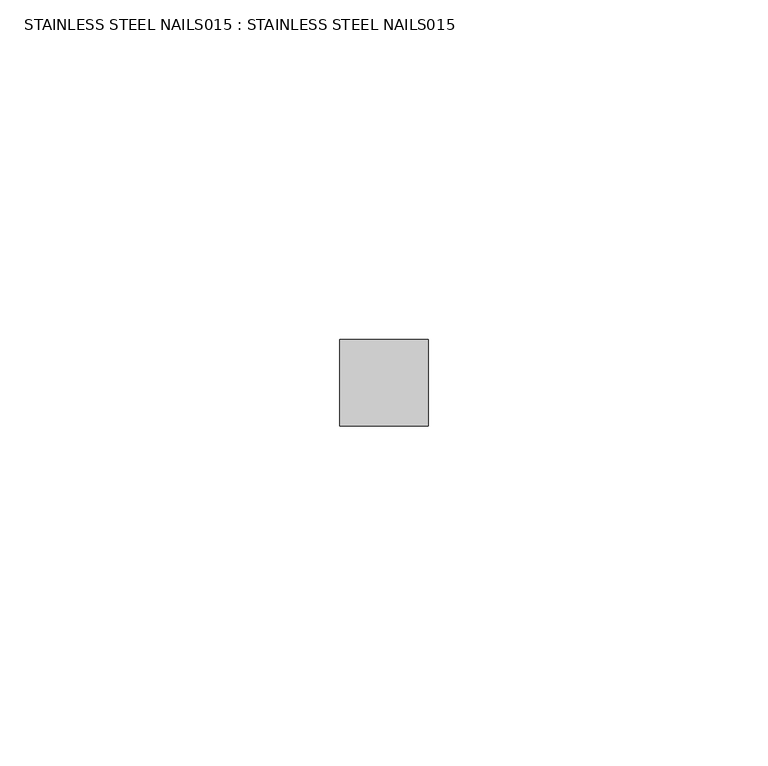
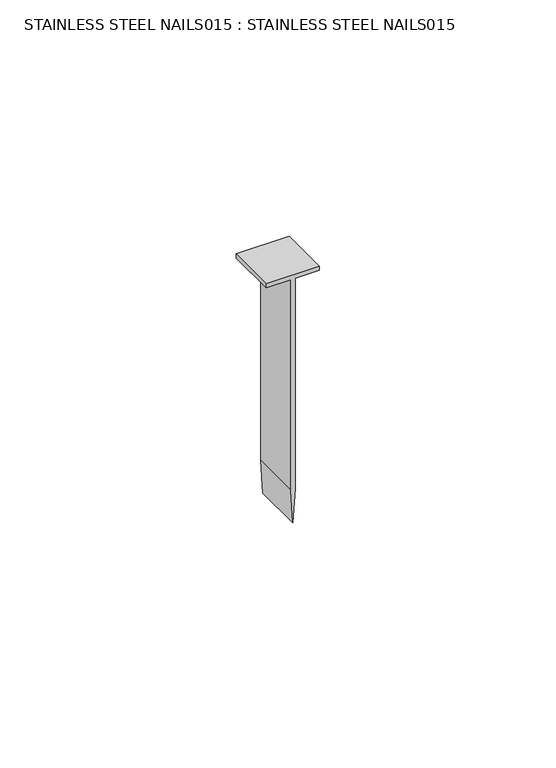
"""IFC4 building model written with IfcOpenShell, lengths in millimetres: proxy geometry, STAINLESS STEEL NAILS015 : STAINLESS STEEL NAILS015."""

from ifc_helpers import new_model, si_unit, frame, origin, place, context, project, spatial, polyline, outline, extrude, source, transform, mapped, element, save


def stainless_steel_nails015_stainless_steel_nails015_84e142ce(model_context):
    return source(origin(), model_context, "Body", "SweptSolid", [
        extrude(outline(polyline([(40259.5998489, -4449.9338534), (40260.6830476, -4449.9338534), (40260.6830476, -4462.9322372), (40259.5998489, -4462.9322372), (40259.5998489, -4456.9746446), (40205.2737053, -4456.9746446), (40196.608116, -4456.4330453), (40205.2737053, -4455.891446), (40259.5998489, -4455.891446), (40259.5998489, -4449.9338534)])), frame((0.0, 934.6593427, 0.0), z_axis=(0.0, 1.0, 0.0), x_axis=(0.0, 0.0, 1.0)), (0.0, 0.0, 1.0), 12.7),
    ])


if __name__ == "__main__":
    model = new_model("IFC4")
    model_context = context("Model", 3, world=origin())
    ifc_project = project(units=[si_unit("LENGTHUNIT", "METRE", prefix="MILLI")], contexts=[model_context])
    site = spatial("IfcSite", under=ifc_project)
    building = spatial("IfcBuilding", under=site)
    placement = place(None, origin())
    stainless_steel_nails015_stainless_steel_nails015_shape = stainless_steel_nails015_stainless_steel_nails015_84e142ce(model_context)
    element("IfcBuildingElementProxy", 1, Name="STAINLESS STEEL NAILS015 : STAINLESS STEEL NAILS015", ObjectType="STAINLESS STEEL NAILS015 : STAINLESS STEEL NAILS015", at=placement, inside=building, context=model_context, shape_type="MappedRepresentation", body=[
        mapped(stainless_steel_nails015_stainless_steel_nails015_shape, transform((0.0, 0.0, 0.0), x_axis=(1.0, 0.0, 0.0), y_axis=(0.0, 1.0, 0.0), z_axis=(0.0, 0.0, 1.0))),
    ])
    save(model, "model.ifc")

# Revit data of these elements
# Type "STAINLESS STEEL NAILS015 : STAINLESS STEEL NAILS015"
#   NameOverride = "STAINLESS STEEL NAILS015"
# Element 1 (IfcBuildingElementProxy, "STAINLESS STEEL NAILS015 : STAINLESS STEEL NAILS015")
#   Materials on its faces: "1 3/4\" STAINLESS STEEL RINGSHANK 5D COMMON NAILS @ 4\" (101.6MM) O.C. FIRESTONE PROVIDED MAX., 1/2\" STAGGERED"
# Materials
#   "1 3/4\" STAINLESS STEEL RINGSHANK 5D COMMON NAILS @ 4\" (101.6MM) O.C. FIRESTONE PROVIDED MAX., 1/2\" STAGGERED": class "Unassigned", colour RGB 255 255 255, transparency 0
